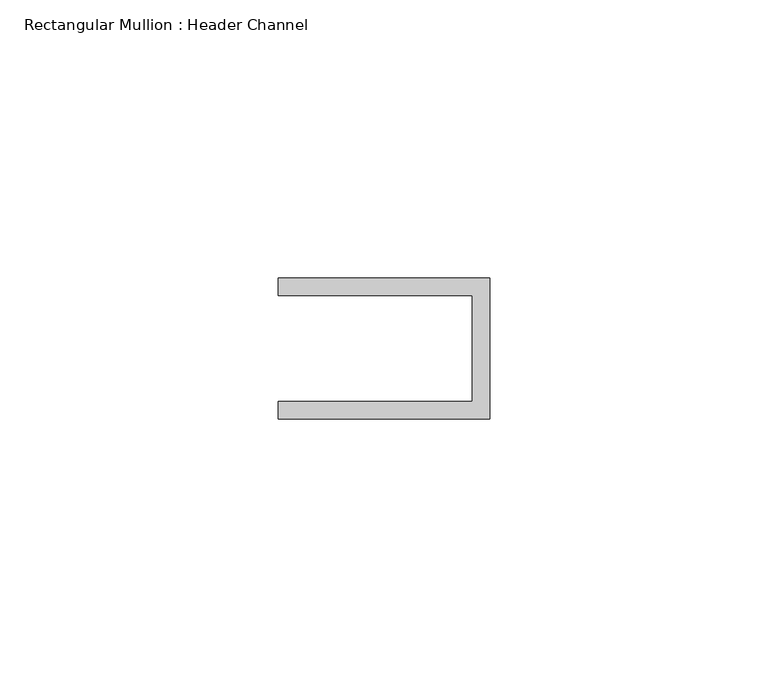
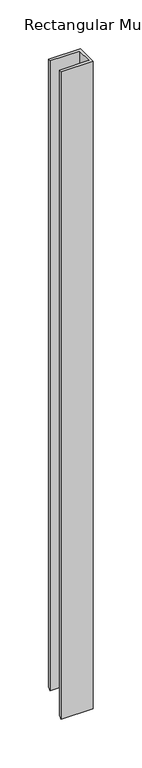
"""IFC4 building model written with IfcOpenShell, lengths in millimetres: member geometry, Rectangular Mullion : Header Channel."""

from ifc_helpers import new_model, si_unit, origin, place, context, project, spatial, faceted_brep, source, transform, mapped, element, save


def rectangular_mullion_header_channel_f191aa13(model_context):
    return source(origin(), model_context, "Body", "Brep", [
        faceted_brep([(0.0, -12.7, 0.0), (0.0, 12.7, 0.0), (-38.1, 12.7, 0.0), (-38.1, 9.525, 0.0), (-3.175, 9.525, 0.0), (-3.175, -9.525, 0.0), (-38.1, -9.525, 0.0), (-38.1, -12.7, 0.0), (0.0, -12.7, -810.1591001), (0.0, 12.7, -784.7591001), (-38.1, 12.7, -784.7591001), (-38.1, 9.525, -787.9341001), (-3.175, 9.525, -787.9341001), (-3.175, -9.525, -806.9841001), (-38.1, -9.525, -806.9841001), (-38.1, -12.7, -810.1591001)], [[[0, 1, 2, 3, 4, 5, 6, 7]], [[1, 0, 8, 9]], [[2, 1, 9, 10]], [[3, 2, 10, 11]], [[4, 3, 11, 12]], [[5, 4, 12, 13]], [[6, 5, 13, 14]], [[7, 6, 14, 15]], [[0, 7, 15, 8]], [[8, 15, 14, 13, 12, 11, 10, 9]]]),
    ])


if __name__ == "__main__":
    model = new_model("IFC4")
    model_context = context("Model", 3, world=origin())
    ifc_project = project(units=[si_unit("LENGTHUNIT", "METRE", prefix="MILLI")], contexts=[model_context])
    site = spatial("IfcSite", under=ifc_project)
    building = spatial("IfcBuilding", under=site)
    placement = place(None, origin())
    rectangular_mullion_header_channel_shape = rectangular_mullion_header_channel_f191aa13(model_context)
    element("IfcMember", 1, ObjectType="Rectangular Mullion : Header Channel", at=placement, inside=building, context=model_context, shape_type="MappedRepresentation", body=[
        mapped(rectangular_mullion_header_channel_shape, transform((0.0, 0.0, 0.0), x_axis=(1.0, 0.0, 0.0), y_axis=(0.0, 1.0, 0.0), z_axis=(0.0, 0.0, 1.0))),
    ])
    save(model, "model.ifc")

# Revit data of these elements
# Type "Rectangular Mullion : Header Channel"
#   built-in parameter 1007322 = 0.0833333 (stored number, unit not read)
#   built-in parameter 1007321 = -0.03125 (stored number, unit not read)
#   built-in parameter 1007320 = 0.0416667 (stored number, unit not read)
# Element 1 (IfcMember, "Rectangular Mullion : Header Channel")
#   Materials on its faces: "ALUM"
# Materials
#   "ALUM": class "Generic", colour RGB 157 157 157, transparency 0, Cost = 0
